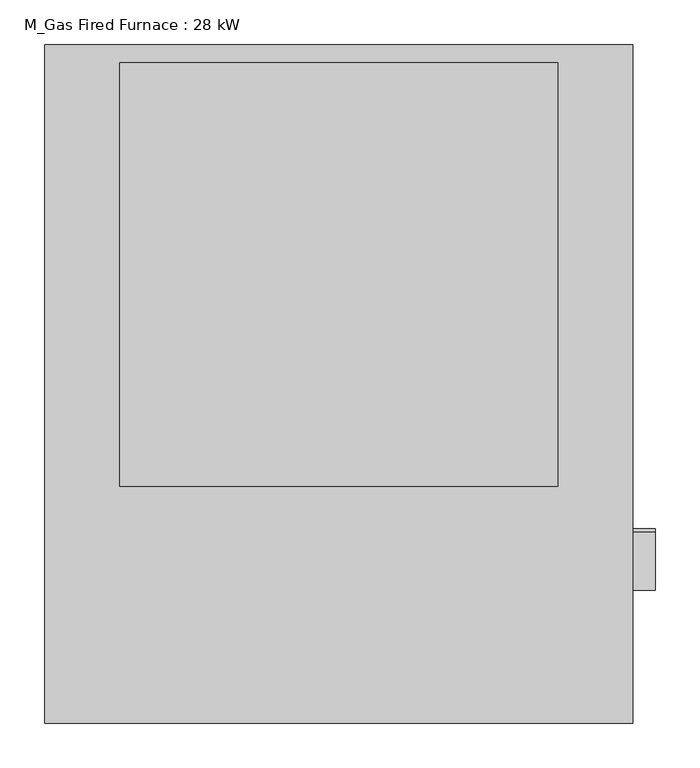
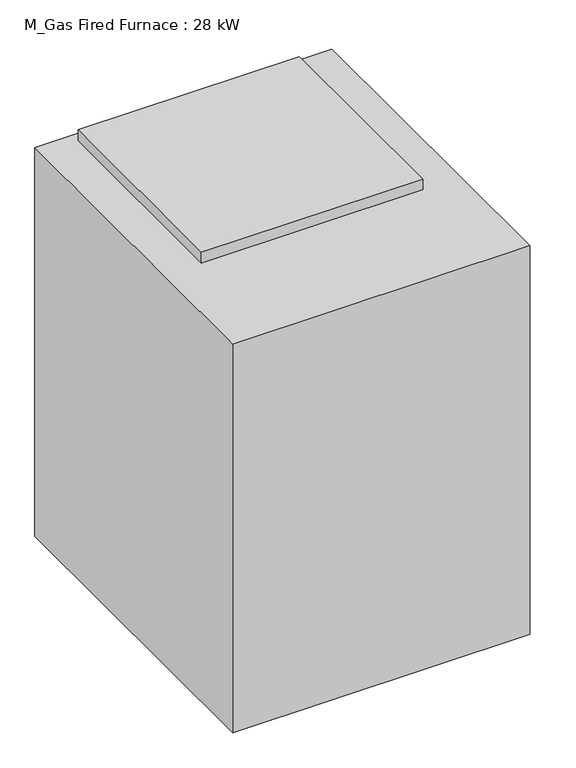
"""IFC4 building model written with IfcOpenShell, lengths in millimetres: proxy geometry, M_Gas Fired Furnace : 28 kW."""

from ifc_helpers import new_model, si_unit, frame, origin, place, context, project, spatial, circle_curve, source, transform, mapped, element, save
from ifc_brep_helpers import plane_surface, cylinder_surface, advanced_brep


def m_gas_fired_furnace_28_kw_1f9757d0(model_context):
    return source(origin(), model_context, "Body", "AdvancedBrep", [
        advanced_brep(
        [(0.0, 0.0, 914.4), (-660.4, 0.0, 914.4), (-660.4, -762.0, 914.4), (0.0, -762.0, 914.4), (-576.2, -20.6375, 914.4), (-84.2, -20.6375, 914.4), (-84.2, -495.6375, 914.4), (-576.2, -495.6375, 914.4), (0.0, 0.0, 0.0), (0.0, -762.0, 0.0), (-660.4, -762.0, 0.0), (-660.4, 0.0, 0.0), (0.0, -547.4666667, 844.55), (0.0, -612.4666667, 844.55), (0.0, -572.4666667, 774.7), (0.0, -587.4666667, 774.7), (0.0, -543.7625, 463.55), (0.0, -608.7625, 463.55), (25.4, -612.4666667, 844.55), (25.4, -547.4666667, 844.55), (25.4, -587.4666667, 774.7), (25.4, -572.4666667, 774.7), (25.4, -608.7625, 463.55), (25.4, -543.7625, 463.55), (-84.2, -20.6375, 939.8), (-576.2, -20.6375, 939.8), (-576.2, -495.6375, 939.8), (-84.2, -495.6375, 939.8)],
        [
            (0, 1),
            (1, 2),
            (2, 3),
            (3, 0),
            (4, 5),
            (5, 6),
            (6, 7),
            (7, 4),
            (8, 9),
            (9, 10),
            (10, 11),
            (11, 8),
            (0, 8),
            (11, 1),
            (10, 2),
            (9, 3),
            (12, 13, circle_curve(frame((0.0, -579.9666667, 844.55), z_axis=(-1.0, 0.0, 0.0), x_axis=(0.0, 1.0, 0.0)), 32.5)),
            (13, 12, circle_curve(frame((0.0, -579.9666667, 844.55), z_axis=(-1.0, 0.0, 0.0), x_axis=(0.0, 1.0, 0.0)), 32.5)),
            (14, 15, circle_curve(frame((0.0, -579.9666667, 774.7), z_axis=(-1.0, 0.0, 0.0), x_axis=(0.0, 1.0, 0.0)), 7.5)),
            (15, 14, circle_curve(frame((0.0, -579.9666667, 774.7), z_axis=(-1.0, 0.0, 0.0), x_axis=(0.0, 1.0, 0.0)), 7.5)),
            (16, 17, circle_curve(frame((0.0, -576.2625, 463.55), z_axis=(-1.0, 0.0, 0.0), x_axis=(0.0, 1.0, 0.0)), 32.5)),
            (17, 16, circle_curve(frame((0.0, -576.2625, 463.55), z_axis=(-1.0, 0.0, 0.0), x_axis=(0.0, 1.0, 0.0)), 32.5)),
            (18, 19, circle_curve(frame((25.4, -579.9666667, 844.55), z_axis=(1.0, 0.0, 0.0), x_axis=(0.0, 1.0, 0.0)), 32.5)),
            (19, 18, circle_curve(frame((25.4, -579.9666667, 844.55), z_axis=(1.0, 0.0, 0.0), x_axis=(0.0, 1.0, 0.0)), 32.5)),
            (20, 21, circle_curve(frame((25.4, -579.9666667, 774.7), z_axis=(1.0, 0.0, 0.0), x_axis=(0.0, 1.0, 0.0)), 7.5)),
            (21, 20, circle_curve(frame((25.4, -579.9666667, 774.7), z_axis=(1.0, 0.0, 0.0), x_axis=(0.0, 1.0, 0.0)), 7.5)),
            (22, 23, circle_curve(frame((25.4, -576.2625, 463.55), z_axis=(1.0, 0.0, 0.0), x_axis=(0.0, 1.0, 0.0)), 32.5)),
            (23, 22, circle_curve(frame((25.4, -576.2625, 463.55), z_axis=(1.0, 0.0, 0.0), x_axis=(0.0, 1.0, 0.0)), 32.5)),
            (18, 13),
            (12, 19),
            (20, 15),
            (14, 21),
            (22, 17),
            (16, 23),
            (24, 25),
            (25, 26),
            (26, 27),
            (27, 24),
            (24, 5),
            (4, 25),
            (7, 26),
            (6, 27),
        ],
        [
            plane_surface(frame((-660.4, 0.0, 914.4), z_axis=(0.0, 0.0, 1.0), x_axis=(-1.0, 0.0, 0.0))),
            plane_surface(frame((-660.4, 0.0, 0.0), z_axis=(0.0, 0.0, -1.0), x_axis=(1.0, 0.0, 0.0))),
            plane_surface(frame((0.0, 0.0, 914.4), z_axis=(0.0, 1.0, 0.0), x_axis=(0.0, 0.0, -1.0))),
            plane_surface(frame((-660.4, 0.0, 914.4), z_axis=(-1.0, 0.0, 0.0), x_axis=(0.0, 0.0, -1.0))),
            plane_surface(frame((-660.4, -762.0, 914.4), z_axis=(0.0, -1.0, 0.0), x_axis=(0.0, 0.0, -1.0))),
            plane_surface(frame((0.0, -762.0, 914.4), z_axis=(1.0, 0.0, 0.0), x_axis=(0.0, 0.0, -1.0))),
            plane_surface(frame((25.4, -547.4666667, 844.55), z_axis=(1.0, 0.0, 0.0), x_axis=(0.0, 0.0, 1.0))),
            cylinder_surface(frame((0.0, -579.9666667, 844.55), z_axis=(1.0, 0.0, 0.0), x_axis=(0.0, 1.0, 0.0)), 32.5),
            cylinder_surface(frame((0.0, -579.9666667, 774.7), z_axis=(1.0, 0.0, 0.0), x_axis=(0.0, 1.0, 0.0)), 7.5),
            cylinder_surface(frame((0.0, -576.2625, 463.55), z_axis=(1.0, 0.0, 0.0), x_axis=(0.0, 1.0, 0.0)), 32.5),
            plane_surface(frame((-576.2, -20.6375, 939.8), z_axis=(0.0, 0.0, 1.0), x_axis=(-1.0, 0.0, 0.0))),
            plane_surface(frame((-84.2, -20.6375, 939.8), z_axis=(0.0, 1.0, 0.0), x_axis=(0.0, 0.0, -1.0))),
            plane_surface(frame((-576.2, -20.6375, 939.8), z_axis=(-1.0, 0.0, 0.0), x_axis=(0.0, 0.0, -1.0))),
            plane_surface(frame((-576.2, -495.6375, 939.8), z_axis=(0.0, -1.0, 0.0), x_axis=(0.0, 0.0, -1.0))),
            plane_surface(frame((-84.2, -495.6375, 939.8), z_axis=(1.0, 0.0, 0.0), x_axis=(0.0, 0.0, -1.0))),
        ],
        [
            (0, [[1, 2, 3, 4], [5, 6, 7, 8]]),
            (1, [[9, 10, 11, 12]]),
            (2, [[-1, 13, -12, 14]]),
            (3, [[-2, -14, -11, 15]]),
            (4, [[-3, -15, -10, 16]]),
            (5, [[-4, -16, -9, -13], [17, 18], [19, 20], [21, 22]]),
            (6, [[23, 24]]),
            (6, [[25, 26]]),
            (6, [[27, 28]]),
            (7, [[-23, 29, -17, 30]]),
            (7, [[-24, -30, -18, -29]]),
            (8, [[-25, 31, -19, 32]]),
            (8, [[-26, -32, -20, -31]]),
            (9, [[-27, 33, -21, 34]]),
            (9, [[-28, -34, -22, -33]]),
            (10, [[35, 36, 37, 38]]),
            (11, [[-35, 39, -5, 40]]),
            (12, [[-36, -40, -8, 41]]),
            (13, [[-37, -41, -7, 42]]),
            (14, [[-38, -42, -6, -39]]),
        ],
    ),
    ])


if __name__ == "__main__":
    model = new_model("IFC4")
    model_context = context("Model", 3, world=origin())
    ifc_project = project(units=[si_unit("LENGTHUNIT", "METRE", prefix="MILLI")], contexts=[model_context])
    site = spatial("IfcSite", under=ifc_project)
    building = spatial("IfcBuilding", under=site)
    placement = place(None, origin())
    m_gas_fired_furnace_28_kw_shape = m_gas_fired_furnace_28_kw_1f9757d0(model_context)
    element("IfcBuildingElementProxy", 1, Name="M_Gas Fired Furnace : 28 kW", ObjectType="M_Gas Fired Furnace : 28 kW", at=placement, inside=building, context=model_context, shape_type="MappedRepresentation", body=[
        mapped(m_gas_fired_furnace_28_kw_shape, transform((0.0, 0.0, 0.0), x_axis=(1.0, 0.0, 0.0), y_axis=(0.0, 1.0, 0.0), z_axis=(0.0, 0.0, 1.0))),
    ])
    save(model, "model.ifc")

# Revit data of these elements
# Project information
#   Project Issue Date = "Issue Date"
#   Project Status = "Project Status"
#   Client Name = "Owner"
#   Project Address = "Enter address here"
#   Project Name = "Lake Geneva"
#   Project Number = "Project Number"
# Type "M_Gas Fired Furnace : 28 kW"
#   Type Mark = "GF-01"
#   dd = 92.1 mm
#   Vent Radius = 1.27953"
#   Vent Diameter = 2.55906"
#   Supply Air Width = 19.37008"
#   Supply Air Height = 18.70079"
#   Return Air Width = 19 1/2"
#   Return Air Height = 24.18898"
#   Output Capacity [instance default] = 93833.9 Btu/h
#   Gas Radius = 0.29528"
#   Gas Pressure Drop [instance default] = 0.00 psi
#   Gas Flow [instance default] = 0 GPM
#   Gas Diameter = 0.59055"
#   Furnace Width = 762 mm
#   Furnace Length = 660.4 mm
#   Furnace Height = 914.4 mm
#   Exhaust Air Pressure Drop [instance default] = 0.00 in-wg
#   Exhaust Air Flow [instance default] = 0 CFM
#   Combustion Air Radius = 1.27953"
#   Combustion Air Pressure Drop [instance default] = 0.00 psi
#   Combustion Air Flow [instance default] = 0 GPM
#   Combustion Air Diameter = 2.55906"
#   Air Pressure Drop [instance default] = 0.00 in-wg
#   Air Flow [instance default] = 2000.22 CFM
#   Material = none
# Element 1 (IfcBuildingElementProxy, "M_Gas Fired Furnace : 28 kW")
#   Output Capacity = 37533.6 Btu/h
#   Air Flow = 1400.58 CFM
